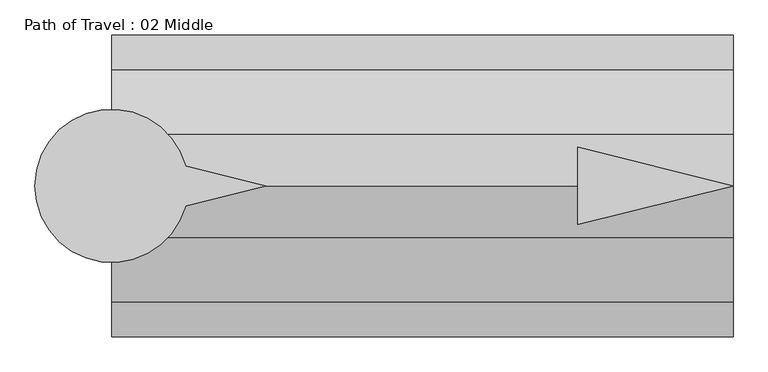
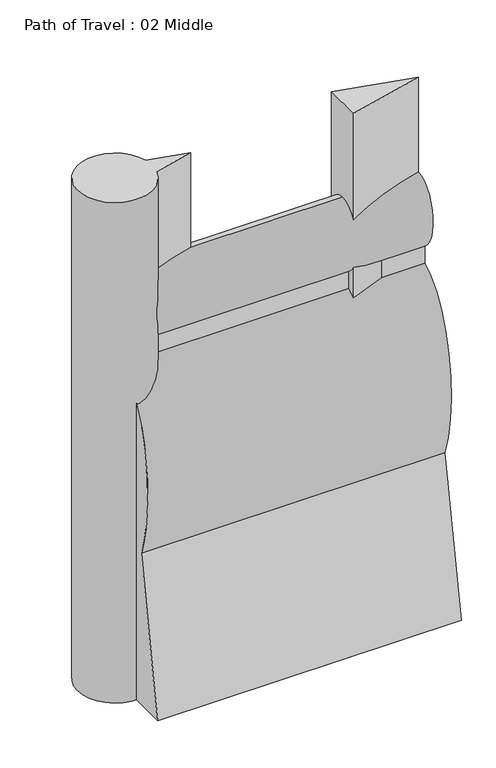
"""IFC4 building model written with IfcOpenShell, lengths in millimetres: proxy geometry, Path of Travel : 02 Middle."""

from ifc_helpers import new_model, si_unit, point, frame, frame_2d, origin, origin_with_axes, place, context, project, spatial, polyline, circle_curve, ellipse_curve, trimmed, segment, composite_curve, outline, extrude, source, transform, mapped, element, save
from ifc_brep_helpers import plane_surface, extruded_surface, advanced_brep


def path_of_travel_02_middle_48d815f7(model_context):
    return source(origin(), model_context, "Body", "SolidModel", [
        advanced_brep(
        [(227.5554837, 0.0, 1727.2), (227.5554837, 42.9018657, 1436.6534209), (227.5554837, 42.9018657, 1363.4763406), (227.5554837, 184.1186263, 643.4144547), (227.5554837, 297.5699544, 0.0), (227.5554837, 145.6574193, 0.0), (227.5554837, 0.0, 584.2), (227.5554837, -145.6574193, 0.0), (227.5554837, -297.5699544, 0.0), (227.5554837, -184.1186263, 643.4144547), (227.5554837, -42.9018657, 1363.4763406), (227.5554837, -42.9018657, 1436.6534209), (1450.4723268, 0.0, 1727.2), (1450.4723268, -42.9018657, 1436.6534209), (1450.4723268, -42.9018657, 1363.4763406), (1450.4723268, -184.1186263, 643.4144547), (1450.4723268, -297.5699544, 0.0), (1450.4723268, -145.6574193, 0.0), (1450.4723268, 0.0, 584.2), (1450.4723268, 145.6574193, 0.0), (1450.4723268, 297.5699544, 0.0), (1450.4723268, 184.1186263, 643.4144547), (1450.4723268, 42.9018657, 1363.4763406), (1450.4723268, 42.9018657, 1436.6534209)],
        [
            (0, 1, ellipse_curve(frame((227.5554837, 0.0, 1574.8), z_axis=(-1.0, 0.0, 0.0), x_axis=(0.0, 0.0, 1.0)), 152.4, 101.6)),
            (1, 2),
            (2, 3, ellipse_curve(frame((227.5554837, 0.0, 914.4), z_axis=(-1.0, 0.0, 0.0), x_axis=(0.0, 0.0, -1.0)), 457.2, 228.6)),
            (3, 4),
            (4, 5),
            (5, 6),
            (6, 7),
            (7, 8),
            (8, 9),
            (9, 10, ellipse_curve(frame((227.5554837, 0.0, 914.4), z_axis=(-1.0, 0.0, 0.0), x_axis=(0.0, 0.0, -1.0)), 457.2, 228.6)),
            (10, 11),
            (11, 0, ellipse_curve(frame((227.5554837, 0.0, 1574.8), z_axis=(-1.0, 0.0, 0.0), x_axis=(0.0, 0.0, 1.0)), 152.4, 101.6)),
            (12, 13, ellipse_curve(frame((1450.4723268, 0.0, 1574.8), z_axis=(1.0, 0.0, 0.0), x_axis=(0.0, 0.0, 1.0)), 152.4, 101.6)),
            (13, 14),
            (14, 15, ellipse_curve(frame((1450.4723268, 0.0, 914.4), z_axis=(1.0, 0.0, 0.0), x_axis=(0.0, 0.0, -1.0)), 457.2, 228.6)),
            (15, 16),
            (16, 17),
            (17, 18),
            (18, 19),
            (19, 20),
            (20, 21),
            (21, 22, ellipse_curve(frame((1450.4723268, 0.0, 914.4), z_axis=(1.0, 0.0, 0.0), x_axis=(0.0, 0.0, -1.0)), 457.2, 228.6)),
            (22, 23),
            (23, 12, ellipse_curve(frame((1450.4723268, 0.0, 1574.8), z_axis=(1.0, 0.0, 0.0), x_axis=(0.0, 0.0, 1.0)), 152.4, 101.6)),
            (0, 12),
            (23, 1),
            (22, 2),
            (21, 3),
            (20, 4),
            (19, 5),
            (18, 6),
            (17, 7),
            (16, 8),
            (15, 9),
            (14, 10),
            (13, 11),
        ],
        [
            plane_surface(frame((227.5554837, 0.0, 0.0), z_axis=(-1.0, 0.0, 0.0), x_axis=(0.0, 0.0, 1.0))),
            plane_surface(frame((1450.4723268, 0.0, 0.0), z_axis=(1.0, 0.0, 0.0), x_axis=(0.0, 0.0, 1.0))),
            extruded_surface(trimmed(ellipse_curve(frame((1450.4723268, 0.0, 1574.8), z_axis=(-1.0, 0.0, 0.0), x_axis=(0.0, 0.0, 1.0)), 152.4, 101.6), [point((1450.4723268, 0.0, 1727.2))], [point((1450.4723268, 42.9018657, 1436.6534209))], True, "CARTESIAN"), (-1222.9168431, 0.0, 0.0), 1222.9168431),
            plane_surface(frame((227.5554837, 42.9018657, 1436.6534209), z_axis=(0.0, 1.0, 0.0), x_axis=(1.0, 0.0, 0.0))),
            extruded_surface(trimmed(ellipse_curve(frame((1450.4723268, 0.0, 914.4), z_axis=(-1.0, 0.0, 0.0), x_axis=(0.0, 0.0, -1.0)), 457.2, 228.6), [point((1450.4723268, 42.9018657, 1363.4763406))], [point((1450.4723268, 184.1186263, 643.4144547))], True, "CARTESIAN"), (-1222.9168431, 0.0, 0.0), 1222.9168431),
            plane_surface(frame((227.5554837, 184.1186263, 643.4144547), z_axis=(0.0, 0.9848077530122078, 0.1736481776669322), x_axis=(1.0, 0.0, 0.0))),
            plane_surface(frame((227.5554837, 297.5699544, 0.0), z_axis=(0.0, 0.0, -1.0), x_axis=(1.0, 0.0, 0.0))),
            plane_surface(frame((227.5554837, 145.6574193, 0.0), z_axis=(0.0, -0.9702957262760199, -0.2419218955995739), x_axis=(1.0, 0.0, 0.0))),
            plane_surface(frame((227.5554837, 0.0, 584.2), z_axis=(0.0, 0.9702957262759961, -0.24192189559966923), x_axis=(1.0, 0.0, 0.0))),
            plane_surface(frame((227.5554837, -145.6574193, 0.0), z_axis=(0.0, 0.0, -1.0), x_axis=(1.0, 0.0, 0.0))),
            plane_surface(frame((227.5554837, -297.5699544, 0.0), z_axis=(0.0, -0.984807753012208, 0.17364817766693066), x_axis=(1.0, 0.0, 0.0))),
            extruded_surface(trimmed(ellipse_curve(frame((1450.4723268, 0.0, 914.4), z_axis=(-1.0, 0.0, 0.0), x_axis=(0.0, 0.0, -1.0)), 457.2, 228.6), [point((1450.4723268, -184.1186263, 643.4144547))], [point((1450.4723268, -42.9018657, 1363.4763406))], True, "CARTESIAN"), (-1222.9168431, 0.0, 0.0), 1222.9168431),
            plane_surface(frame((227.5554837, -42.9018657, 1363.4763406), z_axis=(0.0, -1.0, 0.0), x_axis=(1.0, 0.0, 0.0))),
            extruded_surface(trimmed(ellipse_curve(frame((1450.4723268, 0.0, 1574.8), z_axis=(-1.0, 0.0, 0.0), x_axis=(0.0, 0.0, 1.0)), 152.4, 101.6), [point((1450.4723268, -42.9018657, 1436.6534209))], [point((1450.4723268, 0.0, 1727.2))], True, "CARTESIAN"), (-1222.9168431, 0.0, 0.0), 1222.9168431),
        ],
        [
            (0, [[1, 2, 3, 4, 5, 6, 7, 8, 9, 10, 11, 12]]),
            (1, [[13, 14, 15, 16, 17, 18, 19, 20, 21, 22, 23, 24]]),
            (2, [[-1, 25, -24, 26]]),
            (3, [[-2, -26, -23, 27]]),
            (4, [[-3, -27, -22, 28]]),
            (5, [[-4, -28, -21, 29]]),
            (6, [[-5, -29, -20, 30]]),
            (7, [[-6, -30, -19, 31]]),
            (8, [[-7, -31, -18, 32]]),
            (9, [[-8, -32, -17, 33]]),
            (10, [[-9, -33, -16, 34]]),
            (11, [[-10, -34, -15, 35]]),
            (12, [[-11, -35, -14, 36]]),
            (13, [[-12, -36, -13, -25]]),
        ],
    ),
        extrude(outline(polyline([(1144.4671803, 76.2006338), (1450.4723268, 0.0), (1144.4671803, -76.2006338), (1144.4671803, 76.2006338)])), origin_with_axes(), (0.0, 0.0, 1.0), 2129.5973753),
        extrude(outline(composite_curve([segment(polyline([(372.7837828, 39.4440225), (531.182385, 0.0), (372.7837828, -39.4440225)]), True, "CONTINUOUS"), segment(trimmed(circle_curve(frame_2d((227.2200886, 0.0)), 150.8131956), [point((372.7837828, -39.4440225))], [point((372.7837828, 39.4440225))], False, "CARTESIAN"), True, "CONTINUOUS")], self_intersect=False)), origin_with_axes(), (0.0, 0.0, 1.0), 2129.5973753),
    ])


if __name__ == "__main__":
    model = new_model("IFC4")
    model_context = context("Model", 3, world=origin())
    ifc_project = project(units=[si_unit("LENGTHUNIT", "METRE", prefix="MILLI")], contexts=[model_context])
    site = spatial("IfcSite", under=ifc_project)
    building = spatial("IfcBuilding", under=site)
    placement = place(None, origin())
    path_of_travel_02_middle_shape = path_of_travel_02_middle_48d815f7(model_context)
    element("IfcBuildingElementProxy", 1, Name="Path of Travel : 02 Middle", ObjectType="Path of Travel : 02 Middle", at=placement, inside=building, context=model_context, shape_type="MappedRepresentation", body=[
        mapped(path_of_travel_02_middle_shape, transform((0.0, 0.0, 0.0), x_axis=(1.0, 0.0, 0.0), y_axis=(0.0, 1.0, 0.0), z_axis=(0.0, 0.0, 1.0))),
    ])
    save(model, "model.ifc")

# Revit data of these elements
# Type "Path of Travel : 02 Middle"
#   Path of Egress [instance default] = 4' - 0"
#   built-in parameter 1001306 [instance default] = 4 (stored number, unit not read)
#   Dot at Start = no
#   Arrow in Middle = yes
#   Arrow at End = no
#   Egress Path = none
# Element 1 (IfcBuildingElementProxy, "Path of Travel : 02 Middle")
#   Path of Egress = 4' - 0.14633"
#   built-in parameter 1001306 = 4.01219 (stored number, unit not read)
